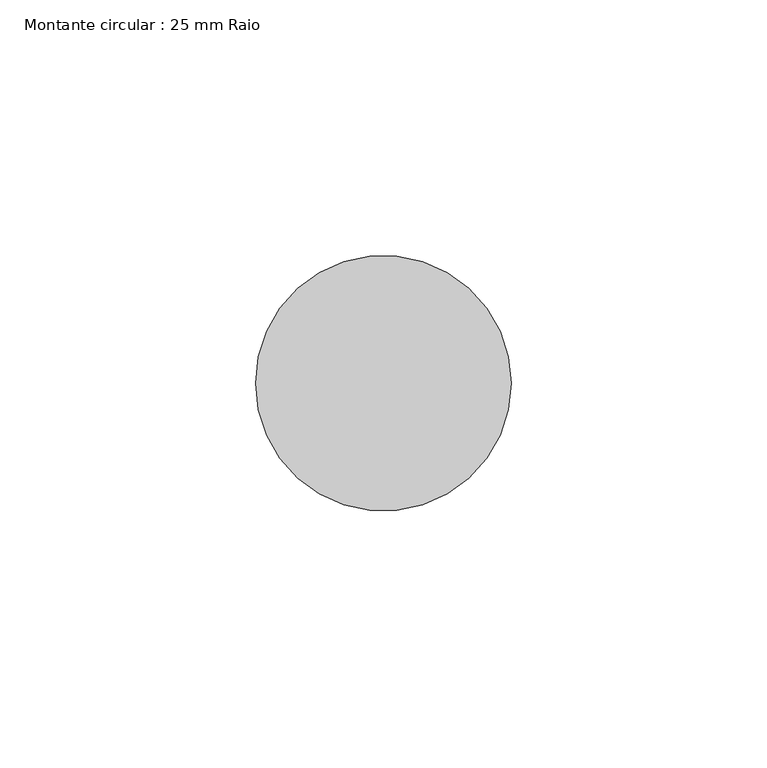
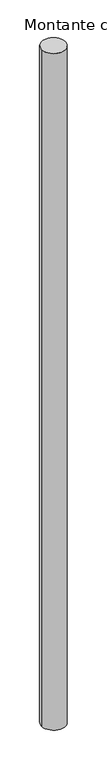
"""IFC4 building model written with IfcOpenShell, lengths in millimetres: member geometry, Montante circular : 25 mm Raio."""

import ifcopenshell
import ifcopenshell.guid

model = None  # the IFC model being written
_history = None  # IfcOwnerHistory: only IFC2X3 demands one
_inside = {}  # id of a spatial element -> (the spatial element, [elements in it])
_under = {}  # id of a project, library or spatial element -> (it, [spatial elements below it])
_declared = {}  # id of a project -> (the project, [libraries it declares])
_typed = {}  # id of a type object -> (the type object, [elements of that type])
_made_of = {}  # id of a material, layer set ... -> (it, [elements and type objects made of it])


def new_model(schema):
    """Start an empty IFC model of exactly this schema.

    Asked for "IFC4X3", IfcOpenShell would pick the latest addendum, in which some entities
    have other attributes; the version numbers below select the first issue.
    IFC2X3 requires an IfcOwnerHistory on every rooted entity: one is made here for all.
    """
    global model, _history
    if schema == "IFC4X3":
        model = ifcopenshell.file(schema_version=(4, 3, 0, 0))
    else:
        model = ifcopenshell.file(schema=schema)
    _inside.clear()
    _under.clear()
    _declared.clear()
    _typed.clear()
    _made_of.clear()
    _history = None
    if model.schema == "IFC2X3":
        org = make("IfcOrganization", Name="unknown")
        user = make(
            "IfcPersonAndOrganization",
            ThePerson=make("IfcPerson", FamilyName="unknown"),
            TheOrganization=org,
        )
        app = make(
            "IfcApplication",
            ApplicationDeveloper=org,
            Version="unknown",
            ApplicationFullName="unknown",
            ApplicationIdentifier="unknown",
        )
        _history = make(
            "IfcOwnerHistory",
            OwningUser=user,
            OwningApplication=app,
            ChangeAction="ADDED",
            CreationDate=0,
        )
    return model


def make(cls, **values):
    """One entity of the class cls with the attributes given. An attribute that is None is left unset."""
    return model.create_entity(
        cls, **{name: value for name, value in values.items() if value is not None}
    )


def rooted(cls, **values):
    """An entity with a GlobalId (a new one), such as an element, a storey or a relation."""
    return make(cls, GlobalId=ifcopenshell.guid.new(), OwnerHistory=_history, **values)


def si_unit(unit_type, name, prefix=None):
    """IfcSIUnit, for example si_unit("LENGTHUNIT", "METRE", prefix="MILLI")."""
    return make("IfcSIUnit", UnitType=unit_type, Prefix=prefix, Name=name)


def assignment(units):
    """IfcUnitAssignment: the units of a project."""
    return None if units is None else make("IfcUnitAssignment", Units=units)


def point(xyz):
    """IfcCartesianPoint."""
    return None if xyz is None else make("IfcCartesianPoint", Coordinates=xyz)


def direction(xyz):
    """IfcDirection."""
    return None if xyz is None else make("IfcDirection", DirectionRatios=xyz)


def frame(location, z_axis=None, x_axis=None):
    """IfcAxis2Placement3D, a coordinate frame: its origin and axes. An axis left out is left unset."""
    return make(
        "IfcAxis2Placement3D",
        Location=point(location),
        Axis=direction(z_axis),
        RefDirection=direction(x_axis),
    )


def frame_2d(location, x_axis=None):
    """IfcAxis2Placement2D, a coordinate frame in the plane: its origin and x axis."""
    return make(
        "IfcAxis2Placement2D", Location=point(location), RefDirection=direction(x_axis)
    )


def origin():
    """The frame at (0, 0, 0) with its axes left unset."""
    return frame((0.0, 0.0, 0.0))


def origin_2d():
    """The frame at (0, 0) in the plane with its x axis left unset."""
    return frame_2d((0.0, 0.0))


def place(relative_to, where):
    """IfcLocalPlacement: puts the frame where relative to a parent placement (None: the world)."""
    return make(
        "IfcLocalPlacement", PlacementRelTo=relative_to, RelativePlacement=where
    )


def context(
    kind, dimensions, precision=None, world=None, true_north=None, identifier=None
):
    """IfcGeometricRepresentationContext, for example the 3D "Model" context."""
    return make(
        "IfcGeometricRepresentationContext",
        ContextIdentifier=identifier,
        ContextType=kind,
        CoordinateSpaceDimension=dimensions,
        Precision=precision,
        WorldCoordinateSystem=world,
        TrueNorth=true_north,
    )


def project(units=None, contexts=None):
    """IfcProject with its units and contexts."""
    return rooted(
        "IfcProject",
        Name="project",
        RepresentationContexts=contexts,
        UnitsInContext=assignment(units),
    )


def spatial(cls, under=None, at=None, **own):
    """A site, building, storey or space (cls), placed at a placement, below another one or the project."""
    s = rooted(cls, ObjectPlacement=at, **own)
    if under is not None:
        _under.setdefault(under.id(), (under, []))[1].append(s)
    return s


def circle_curve(where, radius):
    """IfcCircle in the frame where."""
    return make("IfcCircle", Position=where, Radius=radius)


def trimmed(basis, trim1, trim2, sense, master):
    """IfcTrimmedCurve: the piece of a basis curve between two trims."""
    return make(
        "IfcTrimmedCurve",
        BasisCurve=basis,
        Trim1=trim1,
        Trim2=trim2,
        SenseAgreement=sense,
        MasterRepresentation=master,
    )


def segment(curve, same_sense, transition):
    """IfcCompositeCurveSegment."""
    return make(
        "IfcCompositeCurveSegment",
        Transition=transition,
        SameSense=same_sense,
        ParentCurve=curve,
    )


def composite_curve(segments, self_intersect=None):
    """IfcCompositeCurve: segments joined end to end."""
    return make("IfcCompositeCurve", Segments=segments, SelfIntersect=self_intersect)


def outline(outer, holes=None, kind="AREA"):
    """IfcArbitraryClosedProfileDef: a profile drawn as a closed curve; with holes, ...WithVoids."""
    if holes is None:
        return make("IfcArbitraryClosedProfileDef", ProfileType=kind, OuterCurve=outer)
    return make(
        "IfcArbitraryProfileDefWithVoids",
        ProfileType=kind,
        OuterCurve=outer,
        InnerCurves=holes,
    )


def extrude(swept, where, along, depth):
    """IfcExtrudedAreaSolid: the profile swept, set in the frame where, extruded along a direction by depth."""
    return make(
        "IfcExtrudedAreaSolid",
        SweptArea=swept,
        Position=where,
        ExtrudedDirection=direction(along),
        Depth=depth,
    )


def shape(context_of_items, identifier, shape_type, items):
    """IfcShapeRepresentation: the items that make up one representation, for example the "Body"."""
    return make(
        "IfcShapeRepresentation",
        ContextOfItems=context_of_items,
        RepresentationIdentifier=identifier,
        RepresentationType=shape_type,
        Items=items,
    )


def source(mapping_origin, context_of_items, identifier, shape_type, items):
    """IfcRepresentationMap: a shape defined once, which mapped items show again and again."""
    return make(
        "IfcRepresentationMap",
        MappingOrigin=mapping_origin,
        MappedRepresentation=shape(context_of_items, identifier, shape_type, items),
    )


def transform(
    local_origin,
    x_axis=None,
    y_axis=None,
    z_axis=None,
    scale=None,
    scale2=None,
    scale3=None,
    uniform=True,
):
    """IfcCartesianTransformationOperator3D, or its non-uniform kind. x_axis, y_axis, z_axis: its Axis1, 2, 3."""
    if uniform:
        return make(
            "IfcCartesianTransformationOperator3D",
            Axis1=direction(x_axis),
            Axis2=direction(y_axis),
            LocalOrigin=point(local_origin),
            Scale=scale,
            Axis3=direction(z_axis),
        )
    return make(
        "IfcCartesianTransformationOperator3DnonUniform",
        Axis1=direction(x_axis),
        Axis2=direction(y_axis),
        LocalOrigin=point(local_origin),
        Scale=scale,
        Axis3=direction(z_axis),
        Scale2=scale2,
        Scale3=scale3,
    )


def mapped(mapping_source, mapping_target):
    """IfcMappedItem: shows the shape of a source again, moved by a transform."""
    return make(
        "IfcMappedItem", MappingSource=mapping_source, MappingTarget=mapping_target
    )


def made_of(thing, what):
    """Note that an element or type object is made of a material, layer set ...; save() writes the relation."""
    if what is not None:
        _made_of.setdefault(what.id(), (what, []))[1].append(thing)
    return thing


def element(
    cls,
    number,
    at=None,
    inside=None,
    cuts=None,
    type_object=None,
    material=None,
    context=None,
    identifier="Body",
    shape_type=None,
    held_by="IfcProductDefinitionShape",
    body=None,
    shapes=None,
    **own,
):
    """One element of the class cls, such as IfcWall. Its Tag is "e" and its number.

    at: its placement. inside: the storey or other place that contains it. cuts: it is an
    opening in that element (IfcRelVoidsElement). A single representation is given by context,
    identifier, shape_type and body (its items); several are given by shapes. held_by: the class
    of the entity that holds the representations. save() writes the other relations.
    """
    e = rooted(cls, Tag="e%d" % number, ObjectPlacement=at, **own)
    if body is not None:
        shapes = [shape(context, identifier, shape_type, body)]
    if shapes is not None:
        e.Representation = make(held_by, Representations=shapes)
    if inside is not None:
        _inside.setdefault(inside.id(), (inside, []))[1].append(e)
    if cuts is not None:
        rooted(
            "IfcRelVoidsElement", RelatingBuildingElement=cuts, RelatedOpeningElement=e
        )
    if type_object is not None:
        _typed.setdefault(type_object.id(), (type_object, []))[1].append(e)
    return made_of(e, material)


def aggregate(whole, parts):
    """IfcRelAggregates: a whole, such as a stair, and the parts it consists of."""
    return rooted("IfcRelAggregates", RelatingObject=whole, RelatedObjects=parts)


def save(model, path):
    """Write the relations noted so far, then the file.

    IfcRelAggregates (storeys below a building ...), IfcRelContainedInSpatialStructure (elements
    in a storey), IfcRelDefinesByType, IfcRelAssociatesMaterial and IfcRelDeclares: one each for
    every whole, place, type object, material and project.
    """
    for whole, parts in _under.values():
        aggregate(whole, parts)
    for where, things in _inside.values():
        rooted(
            "IfcRelContainedInSpatialStructure",
            RelatedElements=things,
            RelatingStructure=where,
        )
    for kind, things in _typed.values():
        rooted("IfcRelDefinesByType", RelatedObjects=things, RelatingType=kind)
    for what, things in _made_of.values():
        rooted("IfcRelAssociatesMaterial", RelatedObjects=things, RelatingMaterial=what)
    for by, libraries in _declared.values():
        rooted("IfcRelDeclares", RelatingContext=by, RelatedDefinitions=libraries)
    model.write(path)


def montante_circular_25_mm_raio_36e581cf(model_context):
    return source(origin(), model_context, "Body", "SweptSolid", [
        extrude(outline(composite_curve([segment(trimmed(circle_curve(origin_2d(), 25.0), [point((25.0, 0.0))], [point((-25.0, 0.0))], False, "CARTESIAN"), True, "CONTINUOUS"), segment(trimmed(circle_curve(origin_2d(), 25.0), [point((-25.0, 0.0))], [point((25.0, 0.0))], False, "CARTESIAN"), True, "CONTINUOUS")], self_intersect=False)), frame((0.0, 0.0, -1500.0), z_axis=(0.0, 0.0, 1.0), x_axis=(1.0, 0.0, 0.0)), (0.0, 0.0, 1.0), 1500.0),
    ])


if __name__ == "__main__":
    model = new_model("IFC4")
    model_context = context("Model", 3, world=origin())
    ifc_project = project(units=[si_unit("LENGTHUNIT", "METRE", prefix="MILLI")], contexts=[model_context])
    site = spatial("IfcSite", under=ifc_project)
    building = spatial("IfcBuilding", under=site)
    placement = place(None, origin())
    montante_circular_25_mm_raio_shape = montante_circular_25_mm_raio_36e581cf(model_context)
    element("IfcMember", 1, ObjectType="Montante circular : 25 mm Raio", at=placement, inside=building, context=model_context, shape_type="MappedRepresentation", body=[
        mapped(montante_circular_25_mm_raio_shape, transform((0.0, 0.0, 0.0), x_axis=(1.0, 0.0, 0.0), y_axis=(0.0, 1.0, 0.0), z_axis=(0.0, 0.0, 1.0))),
    ])
    save(model, "model.ifc")

# Revit data of these elements
# Type "Montante circular : 25 mm Raio"
#   built-in parameter 1007350 = 0.082021 (stored number, unit not read)
# Element 1 (IfcMember, "Montante circular : 25 mm Raio")
#   Materials on its faces: "Alumín."
# Materials
#   "Alumín.": class "Metal", colour RGB 247 247 247, transparency 0, Description = "Alumín. 6061", Cost = 0
